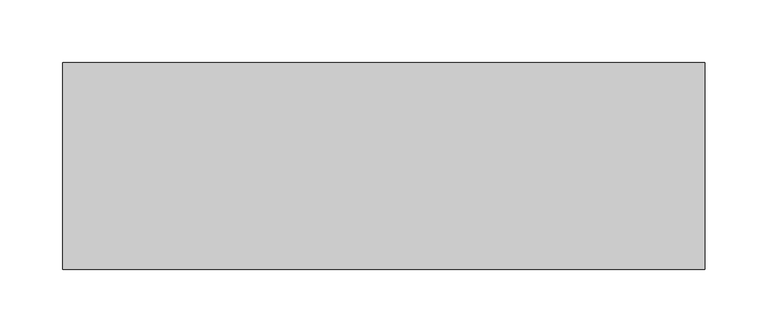
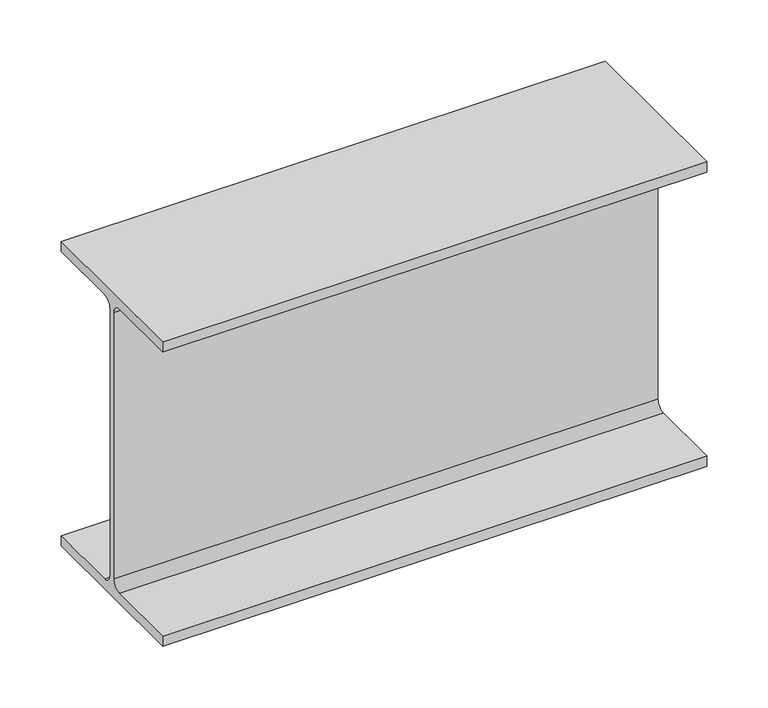
"""IFC4 building model written with IfcOpenShell, lengths in millimetres: beam geometry, Old_Steel Beam_H-KSD3502 : H_SB_ASB_H-300×150x6.5x9."""

import ifcopenshell
import ifcopenshell.guid

model = None  # the IFC model being written
_history = None  # IfcOwnerHistory: only IFC2X3 demands one
_inside = {}  # id of a spatial element -> (the spatial element, [elements in it])
_under = {}  # id of a project, library or spatial element -> (it, [spatial elements below it])
_declared = {}  # id of a project -> (the project, [libraries it declares])
_typed = {}  # id of a type object -> (the type object, [elements of that type])
_made_of = {}  # id of a material, layer set ... -> (it, [elements and type objects made of it])


def new_model(schema):
    """Start an empty IFC model of exactly this schema.

    Asked for "IFC4X3", IfcOpenShell would pick the latest addendum, in which some entities
    have other attributes; the version numbers below select the first issue.
    IFC2X3 requires an IfcOwnerHistory on every rooted entity: one is made here for all.
    """
    global model, _history
    if schema == "IFC4X3":
        model = ifcopenshell.file(schema_version=(4, 3, 0, 0))
    else:
        model = ifcopenshell.file(schema=schema)
    _inside.clear()
    _under.clear()
    _declared.clear()
    _typed.clear()
    _made_of.clear()
    _history = None
    if model.schema == "IFC2X3":
        org = make("IfcOrganization", Name="unknown")
        user = make(
            "IfcPersonAndOrganization",
            ThePerson=make("IfcPerson", FamilyName="unknown"),
            TheOrganization=org,
        )
        app = make(
            "IfcApplication",
            ApplicationDeveloper=org,
            Version="unknown",
            ApplicationFullName="unknown",
            ApplicationIdentifier="unknown",
        )
        _history = make(
            "IfcOwnerHistory",
            OwningUser=user,
            OwningApplication=app,
            ChangeAction="ADDED",
            CreationDate=0,
        )
    return model


def make(cls, **values):
    """One entity of the class cls with the attributes given. An attribute that is None is left unset."""
    return model.create_entity(
        cls, **{name: value for name, value in values.items() if value is not None}
    )


def rooted(cls, **values):
    """An entity with a GlobalId (a new one), such as an element, a storey or a relation."""
    return make(cls, GlobalId=ifcopenshell.guid.new(), OwnerHistory=_history, **values)


def si_unit(unit_type, name, prefix=None):
    """IfcSIUnit, for example si_unit("LENGTHUNIT", "METRE", prefix="MILLI")."""
    return make("IfcSIUnit", UnitType=unit_type, Prefix=prefix, Name=name)


def assignment(units):
    """IfcUnitAssignment: the units of a project."""
    return None if units is None else make("IfcUnitAssignment", Units=units)


def point(xyz):
    """IfcCartesianPoint."""
    return None if xyz is None else make("IfcCartesianPoint", Coordinates=xyz)


def direction(xyz):
    """IfcDirection."""
    return None if xyz is None else make("IfcDirection", DirectionRatios=xyz)


def frame(location, z_axis=None, x_axis=None):
    """IfcAxis2Placement3D, a coordinate frame: its origin and axes. An axis left out is left unset."""
    return make(
        "IfcAxis2Placement3D",
        Location=point(location),
        Axis=direction(z_axis),
        RefDirection=direction(x_axis),
    )


def frame_2d(location, x_axis=None):
    """IfcAxis2Placement2D, a coordinate frame in the plane: its origin and x axis."""
    return make(
        "IfcAxis2Placement2D", Location=point(location), RefDirection=direction(x_axis)
    )


def origin():
    """The frame at (0, 0, 0) with its axes left unset."""
    return frame((0.0, 0.0, 0.0))


def place(relative_to, where):
    """IfcLocalPlacement: puts the frame where relative to a parent placement (None: the world)."""
    return make(
        "IfcLocalPlacement", PlacementRelTo=relative_to, RelativePlacement=where
    )


def context(
    kind, dimensions, precision=None, world=None, true_north=None, identifier=None
):
    """IfcGeometricRepresentationContext, for example the 3D "Model" context."""
    return make(
        "IfcGeometricRepresentationContext",
        ContextIdentifier=identifier,
        ContextType=kind,
        CoordinateSpaceDimension=dimensions,
        Precision=precision,
        WorldCoordinateSystem=world,
        TrueNorth=true_north,
    )


def project(units=None, contexts=None):
    """IfcProject with its units and contexts."""
    return rooted(
        "IfcProject",
        Name="project",
        RepresentationContexts=contexts,
        UnitsInContext=assignment(units),
    )


def spatial(cls, under=None, at=None, **own):
    """A site, building, storey or space (cls), placed at a placement, below another one or the project."""
    s = rooted(cls, ObjectPlacement=at, **own)
    if under is not None:
        _under.setdefault(under.id(), (under, []))[1].append(s)
    return s


def polyline(points):
    """IfcPolyline through the points."""
    return make("IfcPolyline", Points=[point(p) for p in points])


def circle_curve(where, radius):
    """IfcCircle in the frame where."""
    return make("IfcCircle", Position=where, Radius=radius)


def trimmed(basis, trim1, trim2, sense, master):
    """IfcTrimmedCurve: the piece of a basis curve between two trims."""
    return make(
        "IfcTrimmedCurve",
        BasisCurve=basis,
        Trim1=trim1,
        Trim2=trim2,
        SenseAgreement=sense,
        MasterRepresentation=master,
    )


def segment(curve, same_sense, transition):
    """IfcCompositeCurveSegment."""
    return make(
        "IfcCompositeCurveSegment",
        Transition=transition,
        SameSense=same_sense,
        ParentCurve=curve,
    )


def composite_curve(segments, self_intersect=None):
    """IfcCompositeCurve: segments joined end to end."""
    return make("IfcCompositeCurve", Segments=segments, SelfIntersect=self_intersect)


def outline(outer, holes=None, kind="AREA"):
    """IfcArbitraryClosedProfileDef: a profile drawn as a closed curve; with holes, ...WithVoids."""
    if holes is None:
        return make("IfcArbitraryClosedProfileDef", ProfileType=kind, OuterCurve=outer)
    return make(
        "IfcArbitraryProfileDefWithVoids",
        ProfileType=kind,
        OuterCurve=outer,
        InnerCurves=holes,
    )


def extrude(swept, where, along, depth):
    """IfcExtrudedAreaSolid: the profile swept, set in the frame where, extruded along a direction by depth."""
    return make(
        "IfcExtrudedAreaSolid",
        SweptArea=swept,
        Position=where,
        ExtrudedDirection=direction(along),
        Depth=depth,
    )


def shape(context_of_items, identifier, shape_type, items):
    """IfcShapeRepresentation: the items that make up one representation, for example the "Body"."""
    return make(
        "IfcShapeRepresentation",
        ContextOfItems=context_of_items,
        RepresentationIdentifier=identifier,
        RepresentationType=shape_type,
        Items=items,
    )


def source(mapping_origin, context_of_items, identifier, shape_type, items):
    """IfcRepresentationMap: a shape defined once, which mapped items show again and again."""
    return make(
        "IfcRepresentationMap",
        MappingOrigin=mapping_origin,
        MappedRepresentation=shape(context_of_items, identifier, shape_type, items),
    )


def transform(
    local_origin,
    x_axis=None,
    y_axis=None,
    z_axis=None,
    scale=None,
    scale2=None,
    scale3=None,
    uniform=True,
):
    """IfcCartesianTransformationOperator3D, or its non-uniform kind. x_axis, y_axis, z_axis: its Axis1, 2, 3."""
    if uniform:
        return make(
            "IfcCartesianTransformationOperator3D",
            Axis1=direction(x_axis),
            Axis2=direction(y_axis),
            LocalOrigin=point(local_origin),
            Scale=scale,
            Axis3=direction(z_axis),
        )
    return make(
        "IfcCartesianTransformationOperator3DnonUniform",
        Axis1=direction(x_axis),
        Axis2=direction(y_axis),
        LocalOrigin=point(local_origin),
        Scale=scale,
        Axis3=direction(z_axis),
        Scale2=scale2,
        Scale3=scale3,
    )


def mapped(mapping_source, mapping_target):
    """IfcMappedItem: shows the shape of a source again, moved by a transform."""
    return make(
        "IfcMappedItem", MappingSource=mapping_source, MappingTarget=mapping_target
    )


def made_of(thing, what):
    """Note that an element or type object is made of a material, layer set ...; save() writes the relation."""
    if what is not None:
        _made_of.setdefault(what.id(), (what, []))[1].append(thing)
    return thing


def element(
    cls,
    number,
    at=None,
    inside=None,
    cuts=None,
    type_object=None,
    material=None,
    context=None,
    identifier="Body",
    shape_type=None,
    held_by="IfcProductDefinitionShape",
    body=None,
    shapes=None,
    **own,
):
    """One element of the class cls, such as IfcWall. Its Tag is "e" and its number.

    at: its placement. inside: the storey or other place that contains it. cuts: it is an
    opening in that element (IfcRelVoidsElement). A single representation is given by context,
    identifier, shape_type and body (its items); several are given by shapes. held_by: the class
    of the entity that holds the representations. save() writes the other relations.
    """
    e = rooted(cls, Tag="e%d" % number, ObjectPlacement=at, **own)
    if body is not None:
        shapes = [shape(context, identifier, shape_type, body)]
    if shapes is not None:
        e.Representation = make(held_by, Representations=shapes)
    if inside is not None:
        _inside.setdefault(inside.id(), (inside, []))[1].append(e)
    if cuts is not None:
        rooted(
            "IfcRelVoidsElement", RelatingBuildingElement=cuts, RelatedOpeningElement=e
        )
    if type_object is not None:
        _typed.setdefault(type_object.id(), (type_object, []))[1].append(e)
    return made_of(e, material)


def aggregate(whole, parts):
    """IfcRelAggregates: a whole, such as a stair, and the parts it consists of."""
    return rooted("IfcRelAggregates", RelatingObject=whole, RelatedObjects=parts)


def save(model, path):
    """Write the relations noted so far, then the file.

    IfcRelAggregates (storeys below a building ...), IfcRelContainedInSpatialStructure (elements
    in a storey), IfcRelDefinesByType, IfcRelAssociatesMaterial and IfcRelDeclares: one each for
    every whole, place, type object, material and project.
    """
    for whole, parts in _under.values():
        aggregate(whole, parts)
    for where, things in _inside.values():
        rooted(
            "IfcRelContainedInSpatialStructure",
            RelatedElements=things,
            RelatingStructure=where,
        )
    for kind, things in _typed.values():
        rooted("IfcRelDefinesByType", RelatedObjects=things, RelatingType=kind)
    for what, things in _made_of.values():
        rooted("IfcRelAssociatesMaterial", RelatedObjects=things, RelatingMaterial=what)
    for by, libraries in _declared.values():
        rooted("IfcRelDeclares", RelatingContext=by, RelatedDefinitions=libraries)
    model.write(path)


def beam_abe9414c(model_context):
    return source(origin(), model_context, "Body", "SweptSolid", [
        extrude(outline(composite_curve([segment(polyline([(82.5, -141.5), (82.5, -151.7), (-82.5, -151.7), (-82.5, -141.5), (-11.9, -141.5)]), True, "CONTINUOUS"), segment(trimmed(circle_curve(frame_2d((-11.9, -132.6)), 8.9), [point((-11.9, -141.5))], [point((-3.0, -132.6))], True, "CARTESIAN"), True, "CONTINUOUS"), segment(polyline([(-3.0, -132.6), (-3.0, 132.6)]), True, "CONTINUOUS"), segment(trimmed(circle_curve(frame_2d((-11.9, 132.6)), 8.9), [point((-3.0, 132.6))], [point((-11.9, 141.5))], True, "CARTESIAN"), True, "CONTINUOUS"), segment(polyline([(-11.9, 141.5), (-82.5, 141.5), (-82.5, 151.7), (82.5, 151.7), (82.5, 141.5), (11.9, 141.5)]), True, "CONTINUOUS"), segment(trimmed(circle_curve(frame_2d((11.9, 132.6)), 8.9), [point((11.9, 141.5))], [point((3.0, 132.6))], True, "CARTESIAN"), True, "CONTINUOUS"), segment(polyline([(3.0, 132.6), (3.0, -132.6)]), True, "CONTINUOUS"), segment(trimmed(circle_curve(frame_2d((11.9, -132.6)), 8.9), [point((3.0, -132.6))], [point((11.9, -141.5))], True, "CARTESIAN"), True, "CONTINUOUS"), segment(polyline([(11.9, -141.5), (82.5, -141.5)]), True, "CONTINUOUS")], self_intersect=False)), frame((-300.0, 0.0, 0.0), z_axis=(1.0, 0.0, 0.0), x_axis=(0.0, 1.0, 0.0)), (0.0, 0.0, 1.0), 512.3),
    ])


if __name__ == "__main__":
    model = new_model("IFC4")
    model_context = context("Model", 3, world=origin())
    ifc_project = project(units=[si_unit("LENGTHUNIT", "METRE", prefix="MILLI")], contexts=[model_context])
    site = spatial("IfcSite", under=ifc_project)
    building = spatial("IfcBuilding", under=site)
    placement = place(None, origin())
    beam_shape = beam_abe9414c(model_context)
    element("IfcBeam", 1, ObjectType="Old_Steel Beam_H-KSD3502 : H_SB_ASB_H-300×150x6.5x9", at=placement, inside=building, context=model_context, shape_type="MappedRepresentation", body=[
        mapped(beam_shape, transform((0.0, 0.0, 0.0), x_axis=(1.0, 0.0, 0.0), y_axis=(0.0, 1.0, 0.0), z_axis=(0.0, 0.0, 1.0))),
    ])
    save(model, "model.ifc")

# Revit data of these elements
# Type "Old_Steel Beam_H-KSD3502 : H_SB_ASB_H-300×150x6.5x9"
#   Width = 15.0 cm
#   Web Thickness = 0.65 cm
#   Web Fillet = 1.3 cm
#   Warping Constant = 107174.0 cm⁶
#   Torsional Moment of Inertia = 9.9539 cm⁴
#   Torsional Modulus = 1.0 cm³
#   Section Area = 46.78 cm²
#   Plastic Modulus weak axis = 105.0 cm³
#   Plastic Modulus strong axis = 542.0 cm³
#   Perimeter = 1.17 m²/m
#   Nominal Weight = 36.70 kgf/m
#   Moment of Inertia weak axis = 508.00 cm⁴
#   Moment of Inertia strong axis = 7210.00 cm⁴
#   Height = 30.0 cm
#   Flange Thickness = 0.9 cm
#   Elastic Modulus weak axis = 67.7 cm³
#   Elastic Modulus strong axis = 481.0 cm³
#   Centroid Vertical = 15.0 cm
#   Centroid Horizontal = 7.5 cm
#   Length [instance default] = 1.5240 m
#   Structural Material [instance default] = Steel, 45-345
#   Assembly Code = ""
# Element 1 (IfcBeam, "Old_Steel Beam_H-KSD3502 : H_SB_ASB_H-300×150x6.5x9")
#   Structural Material = none
# Materials
#   "Steel, 45-345": class "Metal", colour RGB 189 187 185, transparency 0, Description = "Steel 345 MPa", Cost = 0
